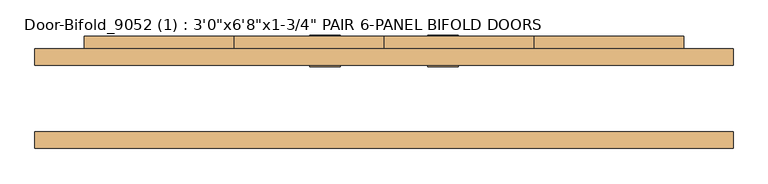
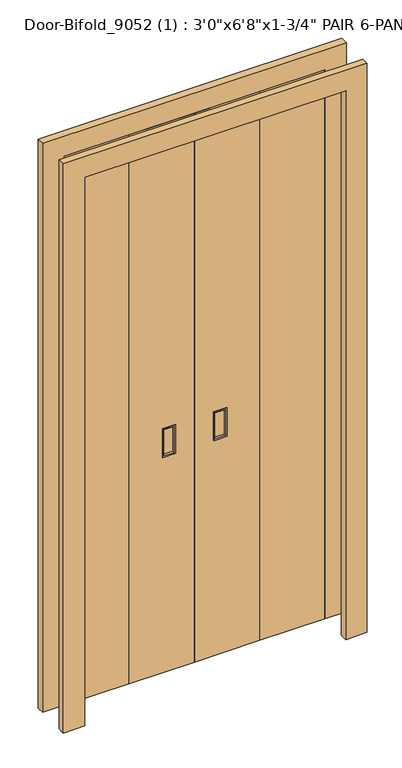
"""IFC4 building model written with IfcOpenShell, lengths in millimetres: door geometry."""

from ifc_helpers import new_model, si_unit, frame, origin, origin_with_axes, place, context, project, spatial, polyline, outline, extrude, faceted_brep, source, transform, mapped, element, save


def door_8ff2f242(model_context):
    return source(origin(), model_context, "Body", "SolidModel", [
        extrude(outline(polyline([(2032.0, -457.2), (2032.0, 457.2), (0.0, 457.2), (0.0, 532.2), (2107.0, 532.2), (2107.0, -532.2), (0.0, -532.2), (0.0, -457.2), (2032.0, -457.2)])), frame((0.0, 50.8, 0.0), z_axis=(0.0, 1.0, 0.0), x_axis=(0.0, 0.0, 1.0)), (0.0, 0.0, 1.0), 25.0),
        extrude(outline(polyline([(2107.0, -532.2), (0.0, -532.2), (0.0, -457.2), (2032.0, -457.2), (2032.0, 457.2), (0.0, 457.2), (0.0, 532.2), (2107.0, 532.2), (2107.0, -532.2)])), frame((0.0, -75.8, 0.0), z_axis=(0.0, 1.0, 0.0), x_axis=(0.0, 0.0, 1.0)), (0.0, 0.0, 1.0), 25.0),
        faceted_brep([(228.6, 50.8, 0.0), (0.0, 50.8, 0.0), (0.0, 95.25, 0.0), (228.6, 95.25, 0.0), (228.6, 50.8, 2032.0), (0.0, 50.8, 2032.0), (110.0, 50.8, 800.0), (70.0, 50.8, 800.0), (70.0, 50.8, 900.0), (110.0, 50.8, 900.0), (0.0, 95.25, 2032.0), (228.6, 95.25, 2032.0), (70.0, 95.25, 800.0), (110.0, 95.25, 800.0), (110.0, 95.25, 900.0), (70.0, 95.25, 900.0), (70.0, 85.25, 800.0), (110.0, 85.25, 800.0), (110.0, 85.25, 900.0), (70.0, 85.25, 900.0), (110.0, 60.8, 800.0), (70.0, 60.8, 800.0), (70.0, 60.8, 900.0), (110.0, 60.8, 900.0)], [[[0, 1, 2, 3]], [[4, 5, 1, 0], [6, 7, 8, 9]], [[5, 10, 2, 1]], [[10, 11, 3, 2], [12, 13, 14, 15]], [[11, 4, 0, 3]], [[16, 17, 13, 12]], [[17, 18, 14, 13]], [[18, 19, 15, 14]], [[19, 16, 12, 15]], [[20, 21, 7, 6]], [[21, 22, 8, 7]], [[22, 23, 9, 8]], [[23, 20, 6, 9]], [[16, 19, 18, 17]], [[20, 23, 22, 21]], [[4, 11, 10, 5]]]),
        faceted_brep([(0.0, 50.8, 0.0), (-228.6, 50.8, 0.0), (-228.6, 95.25, 0.0), (0.0, 95.25, 0.0), (0.0, 50.8, 2032.0), (-228.6, 50.8, 2032.0), (-70.0, 50.8, 900.0), (-70.0, 50.8, 800.0), (-110.0, 50.8, 800.0), (-110.0, 50.8, 900.0), (-228.6, 95.25, 2032.0), (0.0, 95.25, 2032.0), (-110.0, 95.25, 800.0), (-70.0, 95.25, 800.0), (-70.0, 95.25, 900.0), (-110.0, 95.25, 900.0), (-110.0, 85.25, 800.0), (-70.0, 85.25, 800.0), (-70.0, 85.25, 900.0), (-110.0, 85.25, 900.0), (-70.0, 60.8, 900.0), (-70.0, 60.8, 800.0), (-110.0, 60.8, 800.0), (-110.0, 60.8, 900.0)], [[[0, 1, 2, 3]], [[4, 5, 1, 0], [6, 7, 8, 9]], [[5, 10, 2, 1]], [[10, 11, 3, 2], [12, 13, 14, 15]], [[11, 4, 0, 3]], [[16, 17, 13, 12]], [[17, 18, 14, 13]], [[18, 19, 15, 14]], [[19, 16, 12, 15]], [[20, 21, 7, 6]], [[21, 22, 8, 7]], [[22, 23, 9, 8]], [[23, 20, 6, 9]], [[16, 19, 18, 17]], [[20, 23, 22, 21]], [[4, 11, 10, 5]]]),
        extrude(outline(polyline([(457.2, 95.25), (457.2, 50.8), (228.6, 50.8), (228.6, 95.25), (457.2, 95.25)])), origin_with_axes(), (0.0, 0.0, 1.0), 2032.0),
        extrude(outline(polyline([(-228.6, 95.25), (-228.6, 50.8), (-457.2, 50.8), (-457.2, 95.25), (-228.6, 95.25)])), origin_with_axes(), (0.0, 0.0, 1.0), 2032.0),
        extrude(outline(polyline([(108.0022505, 57.666881), (71.9977495, 57.666881), (71.9977495, 60.8), (108.0022505, 60.8), (108.0022505, 57.666881)])), frame((0.0, 0.0, 801.9977495), z_axis=(0.0, 0.0, 1.0), x_axis=(1.0, 0.0, 0.0)), (0.0, 0.0, 1.0), 96.004501),
        faceted_brep([(110.0, 60.8, 800.0), (110.0, 50.8, 800.0), (70.0, 50.8, 800.0), (70.0, 60.8, 800.0), (108.0022505, 48.8449345, 801.9977495), (108.0022505, 60.8, 801.9977495), (71.9977495, 60.8, 801.9977495), (71.9977495, 48.8449345, 801.9977495), (113.0022505, 50.8, 796.9977495), (113.0022505, 48.8449345, 796.9977495), (66.9977495, 48.8449345, 796.9977495), (66.9977495, 50.8, 796.9977495), (70.0, 50.8, 900.0), (70.0, 60.8, 900.0), (71.9977495, 60.8, 898.0022505), (71.9977495, 48.8449345, 898.0022505), (66.9977495, 48.8449345, 903.0022505), (66.9977495, 50.8, 903.0022505), (110.0, 50.8, 900.0), (110.0, 60.8, 900.0), (108.0022505, 60.8, 898.0022505), (108.0022505, 48.8449345, 898.0022505), (113.0022505, 48.8449345, 903.0022505), (113.0022505, 50.8, 903.0022505)], [[[0, 1, 2, 3]], [[4, 5, 6, 7]], [[8, 9, 10, 11]], [[3, 2, 12, 13]], [[7, 6, 14, 15]], [[11, 10, 16, 17]], [[13, 12, 18, 19]], [[15, 14, 20, 21]], [[17, 16, 22, 23]], [[11, 17, 23, 8], [1, 18, 12, 2]], [[19, 18, 1, 0]], [[3, 13, 19, 0], [5, 20, 14, 6]], [[21, 20, 5, 4]], [[9, 22, 16, 10], [7, 15, 21, 4]], [[23, 22, 9, 8]]]),
        extrude(outline(polyline([(-108.0022505, 60.8), (-71.9977495, 60.8), (-71.9977495, 57.666881), (-108.0022505, 57.666881), (-108.0022505, 60.8)])), frame((0.0, 0.0, 801.9977495), z_axis=(0.0, 0.0, 1.0), x_axis=(1.0, 0.0, 0.0)), (0.0, 0.0, 1.0), 96.004501),
        faceted_brep([(-70.0, 60.8, 800.0), (-70.0, 50.8, 800.0), (-110.0, 50.8, 800.0), (-110.0, 60.8, 800.0), (-71.9977495, 48.8449345, 801.9977495), (-71.9977495, 60.8, 801.9977495), (-108.0022505, 60.8, 801.9977495), (-108.0022505, 48.8449345, 801.9977495), (-66.9977495, 50.8, 796.9977495), (-66.9977495, 48.8449345, 796.9977495), (-113.0022505, 48.8449345, 796.9977495), (-113.0022505, 50.8, 796.9977495), (-110.0, 50.8, 900.0), (-110.0, 60.8, 900.0), (-108.0022505, 60.8, 898.0022505), (-108.0022505, 48.8449345, 898.0022505), (-113.0022505, 48.8449345, 903.0022505), (-113.0022505, 50.8, 903.0022505), (-70.0, 50.8, 900.0), (-70.0, 60.8, 900.0), (-71.9977495, 60.8, 898.0022505), (-71.9977495, 48.8449345, 898.0022505), (-66.9977495, 48.8449345, 903.0022505), (-66.9977495, 50.8, 903.0022505)], [[[0, 1, 2, 3]], [[4, 5, 6, 7]], [[8, 9, 10, 11]], [[3, 2, 12, 13]], [[7, 6, 14, 15]], [[11, 10, 16, 17]], [[13, 12, 18, 19]], [[15, 14, 20, 21]], [[17, 16, 22, 23]], [[11, 17, 23, 8], [1, 18, 12, 2]], [[19, 18, 1, 0]], [[3, 13, 19, 0], [5, 20, 14, 6]], [[21, 20, 5, 4]], [[9, 22, 16, 10], [7, 15, 21, 4]], [[23, 22, 9, 8]]]),
        extrude(outline(polyline([(-71.9977495, 85.25), (-108.0022505, 85.25), (-108.0022505, 88.5598365), (-71.9977495, 88.5598365), (-71.9977495, 85.25)])), frame((0.0, 0.0, 801.9977495), z_axis=(0.0, 0.0, 1.0), x_axis=(1.0, 0.0, 0.0)), (0.0, 0.0, 1.0), 96.004501),
        extrude(outline(polyline([(108.0022505, 85.25), (71.9977495, 85.25), (71.9977495, 88.5598365), (108.0022505, 88.5598365), (108.0022505, 85.25)])), frame((0.0, 0.0, 801.9977495), z_axis=(0.0, 0.0, 1.0), x_axis=(1.0, 0.0, 0.0)), (0.0, 0.0, 1.0), 96.004501),
        faceted_brep([(110.0, 85.25, 900.0), (110.0, 95.25, 900.0), (70.0, 95.25, 900.0), (70.0, 85.25, 900.0), (108.0022505, 97.2050655, 898.0022505), (108.0022505, 85.25, 898.0022505), (71.9977495, 85.25, 898.0022505), (71.9977495, 97.2050655, 898.0022505), (113.0022505, 95.25, 903.0022505), (113.0022505, 97.2050655, 903.0022505), (66.9977495, 97.2050655, 903.0022505), (66.9977495, 95.25, 903.0022505), (70.0, 95.25, 800.0), (70.0, 85.25, 800.0), (71.9977495, 85.25, 801.9977495), (71.9977495, 97.2050655, 801.9977495), (66.9977495, 97.2050655, 796.9977495), (66.9977495, 95.25, 796.9977495), (110.0, 95.25, 800.0), (110.0, 85.25, 800.0), (108.0022505, 85.25, 801.9977495), (108.0022505, 97.2050655, 801.9977495), (113.0022505, 97.2050655, 796.9977495), (113.0022505, 95.25, 796.9977495)], [[[0, 1, 2, 3]], [[4, 5, 6, 7]], [[8, 9, 10, 11]], [[3, 2, 12, 13]], [[7, 6, 14, 15]], [[11, 10, 16, 17]], [[13, 12, 18, 19]], [[15, 14, 20, 21]], [[17, 16, 22, 23]], [[11, 17, 23, 8], [1, 18, 12, 2]], [[19, 18, 1, 0]], [[3, 13, 19, 0], [5, 20, 14, 6]], [[21, 20, 5, 4]], [[9, 22, 16, 10], [7, 15, 21, 4]], [[23, 22, 9, 8]]]),
        faceted_brep([(-70.0, 85.25, 900.0), (-70.0, 95.25, 900.0), (-110.0, 95.25, 900.0), (-110.0, 85.25, 900.0), (-71.9977495, 97.2050655, 898.0022505), (-71.9977495, 85.25, 898.0022505), (-108.0022505, 85.25, 898.0022505), (-108.0022505, 97.2050655, 898.0022505), (-66.9977495, 95.25, 903.0022505), (-66.9977495, 97.2050655, 903.0022505), (-113.0022505, 97.2050655, 903.0022505), (-113.0022505, 95.25, 903.0022505), (-110.0, 95.25, 800.0), (-110.0, 85.25, 800.0), (-108.0022505, 85.25, 801.9977495), (-108.0022505, 97.2050655, 801.9977495), (-113.0022505, 97.2050655, 796.9977495), (-113.0022505, 95.25, 796.9977495), (-70.0, 95.25, 800.0), (-70.0, 85.25, 800.0), (-71.9977495, 85.25, 801.9977495), (-71.9977495, 97.2050655, 801.9977495), (-66.9977495, 97.2050655, 796.9977495), (-66.9977495, 95.25, 796.9977495)], [[[0, 1, 2, 3]], [[4, 5, 6, 7]], [[8, 9, 10, 11]], [[3, 2, 12, 13]], [[7, 6, 14, 15]], [[11, 10, 16, 17]], [[13, 12, 18, 19]], [[15, 14, 20, 21]], [[17, 16, 22, 23]], [[11, 17, 23, 8], [1, 18, 12, 2]], [[19, 18, 1, 0]], [[3, 13, 19, 0], [5, 20, 14, 6]], [[21, 20, 5, 4]], [[9, 22, 16, 10], [7, 15, 21, 4]], [[23, 22, 9, 8]]]),
    ])


if __name__ == "__main__":
    model = new_model("IFC4")
    model_context = context("Model", 3, world=origin())
    ifc_project = project(units=[si_unit("LENGTHUNIT", "METRE", prefix="MILLI")], contexts=[model_context])
    site = spatial("IfcSite", under=ifc_project)
    building = spatial("IfcBuilding", under=site)
    placement = place(None, origin())
    door_shape = door_8ff2f242(model_context)
    element("IfcDoor", 1, ObjectType="Door-Bifold_9052 (1) : 3'0\"x6'8\"x1-3/4\" PAIR 6-PANEL BIFOLD DOORS", at=placement, inside=building, context=model_context, shape_type="MappedRepresentation", body=[
        mapped(door_shape, transform((0.0, 0.0, 0.0), x_axis=(1.0, 0.0, 0.0), y_axis=(0.0, 1.0, 0.0), z_axis=(0.0, 0.0, 1.0))),
    ])
    save(model, "model.ifc")

# Revit data of these elements
# Type "Door-Bifold_9052 (1) : 3'0\"x6'8\"x1-3/4\" PAIR 6-PANEL BIFOLD DOORS"
#   Type Mark = "26"
#   Model = "Porta de Fole"
#   Manufacturer = "Typhoon"
#   Thickness = 0' - 1 3/4"
#   Frame Projection Ext. = 0' - 0.98425"
#   Frame Projection Int. = 0' - 0.98425"
#   Frame Width = 0' - 2.95276"
#   Height = 6' - 8"
#   Width = 3' - 0"
#   Comp_painel = 0' - 9"
#   Abertura = 0.00°
#   Altura Puxador = 2' - 11.43307"
#   Puxador = Puxador
#   Painel-Porta = Porta-Painel
#   Function = (empty or 0)
#   Wall Closure = (empty or 0)
# Element 1 (IfcDoor, "Door-Bifold_9052 (1) : 3'0\"x6'8\"x1-3/4\" PAIR 6-PANEL BIFOLD DOORS")
#   Materials on its faces: "Puxador", "Porta-Painel"
# Materials
#   "Puxador": class "Metal", colour RGB 244 244 244, transparency 0
#   "Porta-Painel": class "Wood", colour RGB 135 74 45, transparency 0
